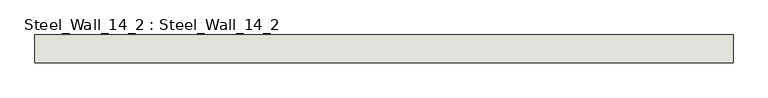
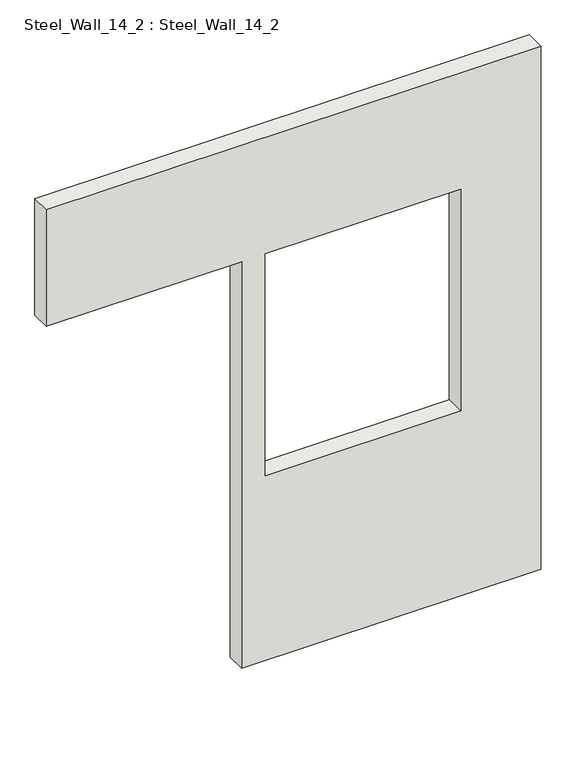
"""IFC4 building model written with IfcOpenShell, lengths in millimetres: wall geometry, Steel_Wall_14_2 : Steel_Wall_14_2."""

from ifc_helpers import new_model, si_unit, frame, origin, place, context, project, spatial, polyline, outline, extrude, source, transform, mapped, element, save


def steel_wall_14_2_steel_wall_14_2_555e5885(model_context):
    return source(origin(), model_context, "Body", "SweptSolid", [
        extrude(outline(polyline([(3080.0, 3460.0), (3080.0, 930.0), (2450.0, 930.0), (2450.0, 1930.0), (250.0, 1930.0), (250.0, 3460.0), (3080.0, 3460.0)]), holes=[polyline([(2450.0, 2050.0), (2450.0, 3050.0), (1250.0, 3050.0), (1250.0, 2050.0), (2450.0, 2050.0)])]), frame((0.0, 395.0, 0.0), z_axis=(0.0, 1.0, 0.0), x_axis=(0.0, 0.0, 1.0)), (0.0, 0.0, 1.0), 100.0),
    ])


if __name__ == "__main__":
    model = new_model("IFC4")
    model_context = context("Model", 3, world=origin())
    ifc_project = project(units=[si_unit("LENGTHUNIT", "METRE", prefix="MILLI")], contexts=[model_context])
    site = spatial("IfcSite", under=ifc_project)
    building = spatial("IfcBuilding", under=site)
    placement = place(None, origin())
    steel_wall_14_2_steel_wall_14_2_shape = steel_wall_14_2_steel_wall_14_2_555e5885(model_context)
    element("IfcWall", 1, ObjectType="Steel_Wall_14_2 : Steel_Wall_14_2", at=placement, inside=building, context=model_context, shape_type="MappedRepresentation", body=[
        mapped(steel_wall_14_2_steel_wall_14_2_shape, transform((0.0, 0.0, 0.0), x_axis=(1.0, 0.0, 0.0), y_axis=(0.0, 1.0, 0.0), z_axis=(0.0, 0.0, 1.0))),
    ])
    save(model, "model.ifc")

# Revit data of these elements
# Type "Steel_Wall_14_2 : Steel_Wall_14_2"
#   NameOverride = "Steel_Wall_14_2"
# Element 1 (IfcWall, "Steel_Wall_14_2 : Steel_Wall_14_2")
#   Materials on its faces: "IfcSurfaceStyle #33"
# Materials
#   "IfcSurfaceStyle #33": class "Unassigned", colour RGB 214 214 214, transparency 0
